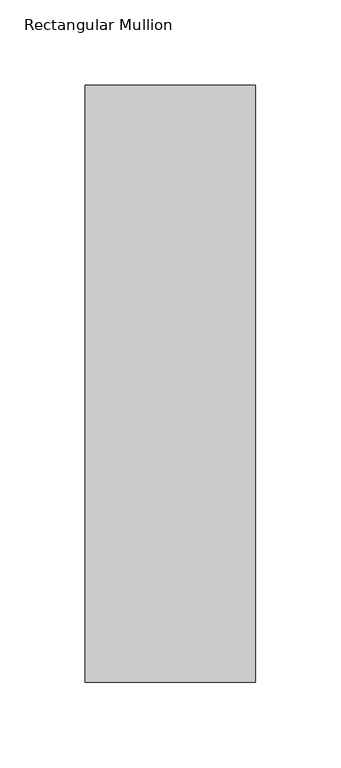
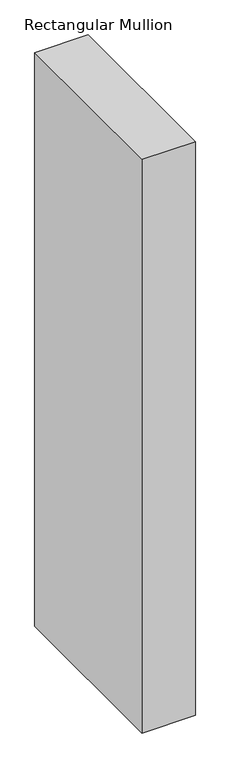
"""IFC4 building model written with IfcOpenShell, lengths in millimetres: member geometry, Rectangular Mullion : WWm-100x350-100mmOffset."""

from ifc_helpers import new_model, si_unit, frame, origin, place, context, project, spatial, polyline, outline, extrude, source, transform, mapped, element, save


def rectangular_mullion_1c8133e1(model_context):
    return source(origin(), model_context, "Body", "SweptSolid", [
        extrude(outline(polyline([(0.0, 175.0), (0.0, -175.0), (-100.0, -175.0), (-100.0, 175.0), (0.0, 175.0)])), frame((0.0, 0.0, -1141.0342645), z_axis=(0.0, 0.0, 1.0), x_axis=(1.0, 0.0, 0.0)), (0.0, 0.0, 1.0), 1141.0342645),
    ])


if __name__ == "__main__":
    model = new_model("IFC4")
    model_context = context("Model", 3, world=origin())
    ifc_project = project(units=[si_unit("LENGTHUNIT", "METRE", prefix="MILLI")], contexts=[model_context])
    site = spatial("IfcSite", under=ifc_project)
    building = spatial("IfcBuilding", under=site)
    placement = place(None, origin())
    rectangular_mullion_shape = rectangular_mullion_1c8133e1(model_context)
    element("IfcMember", 1, ObjectType="Rectangular Mullion : WWm-100x350-100mmOffset", at=placement, inside=building, context=model_context, shape_type="MappedRepresentation", body=[
        mapped(rectangular_mullion_shape, transform((0.0, 0.0, 0.0), x_axis=(1.0, 0.0, 0.0), y_axis=(0.0, 1.0, 0.0), z_axis=(0.0, 0.0, 1.0))),
    ])
    save(model, "model.ifc")

# Revit data of these elements
# Type "Rectangular Mullion : WWm-100x350-100mmOffset"
#   built-in parameter 1007304 = 1.14829 (stored number, unit not read)
#   built-in parameter 1007301 = 0.164042 (stored number, unit not read)
#   built-in parameter 1007300 = 0.164042 (stored number, unit not read)
# Element 1 (IfcMember, "Rectangular Mullion : WWm-100x350-100mmOffset")
#   Materials on its faces: "WW-EC-RGB-Mullion"
# Materials
#   "WW-EC-RGB-Mullion": class "Generic", colour RGB 255 255 255, transparency 0, Comments = "If region requests black mullions, switch asset color to RGB 25-25-25", Description = "Generic Color", Cost = 0
